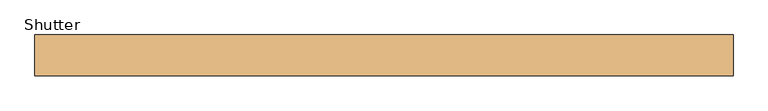
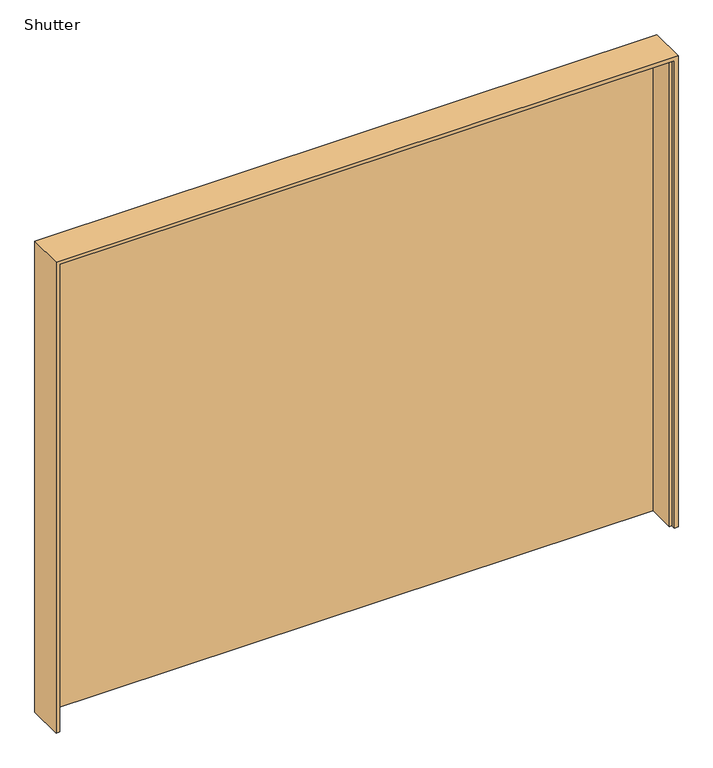
"""IFC4 building model written with IfcOpenShell, lengths in millimetres: door geometry, Shutter : H_DR_AMB_Roll up Door_Steel_W5000xH4000_Motorized."""

from ifc_helpers import new_model, si_unit, origin, origin_with_axes, place, context, project, spatial, polyline, outline, extrude, faceted_brep, source, transform, mapped, element, save


def shutter_f4e91935(model_context):
    return source(origin(), model_context, "Body", "SolidModel", [
        extrude(outline(polyline([(2470.0, 147.0), (2470.0, 112.0), (-2470.0, 112.0), (-2470.0, 147.0), (2470.0, 147.0)])), origin_with_axes(), (0.0, 0.0, 1.0), 3970.0),
        faceted_brep([(2470.0, 147.0, 0.0), (2500.0, 147.0, 0.0), (2500.0, -147.0, 0.0), (2470.0, -147.0, 0.0), (2470.0, -112.0, 0.0), (2450.0, -112.0, 0.0), (2450.0, 112.0, 0.0), (2470.0, 112.0, 0.0), (2470.0, 147.0, 3970.0), (-2470.0, 147.0, 3970.0), (-2470.0, 147.0, 0.0), (-2500.0, 147.0, 0.0), (-2500.0, 147.0, 4000.0), (2500.0, 147.0, 4000.0), (2500.0, -147.0, 4000.0), (-2500.0, -147.0, 4000.0), (-2500.0, -147.0, 0.0), (-2470.0, -147.0, 0.0), (-2470.0, -147.0, 3970.0), (2470.0, -147.0, 3970.0), (2470.0, -112.0, 3970.0), (-2470.0, -112.0, 3970.0), (-2470.0, -112.0, 0.0), (-2450.0, -112.0, 0.0), (-2450.0, -112.0, 3950.0), (2450.0, -112.0, 3950.0), (2450.0, 112.0, 3950.0), (-2450.0, 112.0, 3950.0), (-2450.0, 112.0, 0.0), (-2470.0, 112.0, 0.0), (-2470.0, 112.0, 3970.0), (2470.0, 112.0, 3970.0)], [[[0, 1, 2, 3, 4, 5, 6, 7]], [[1, 0, 8, 9, 10, 11, 12, 13]], [[2, 1, 13, 14]], [[3, 2, 14, 15, 16, 17, 18, 19]], [[4, 3, 19, 20]], [[5, 4, 20, 21, 22, 23, 24, 25]], [[6, 5, 25, 26]], [[7, 6, 26, 27, 28, 29, 30, 31]], [[0, 7, 31, 8]], [[9, 30, 29, 10]], [[10, 29, 28, 23, 22, 17, 16, 11]], [[15, 12, 11, 16]], [[21, 18, 17, 22]], [[27, 24, 23, 28]], [[8, 31, 30, 9]], [[14, 13, 12, 15]], [[20, 19, 18, 21]], [[26, 25, 24, 27]]]),
    ])


if __name__ == "__main__":
    model = new_model("IFC4")
    model_context = context("Model", 3, world=origin())
    ifc_project = project(units=[si_unit("LENGTHUNIT", "METRE", prefix="MILLI")], contexts=[model_context])
    site = spatial("IfcSite", under=ifc_project)
    building = spatial("IfcBuilding", under=site)
    placement = place(None, origin())
    shutter_shape = shutter_f4e91935(model_context)
    element("IfcDoor", 1, ObjectType="Shutter : H_DR_AMB_Roll up Door_Steel_W5000xH4000_Motorized", at=placement, inside=building, context=model_context, shape_type="MappedRepresentation", body=[
        mapped(shutter_shape, transform((0.0, 0.0, 0.0), x_axis=(1.0, 0.0, 0.0), y_axis=(0.0, 1.0, 0.0), z_axis=(0.0, 0.0, 1.0))),
    ])
    save(model, "model.ifc")

# Revit data of these elements
# Type "Shutter : H_DR_AMB_Roll up Door_Steel_W5000xH4000_Motorized"
#   Type Mark = "363"
#   Analytic Construction = "<None>"
#   프레임 투영 외부. = 25 mm
#   프레임 투영 내부. = 25 mm
#   프레임 폭 = 75 mm
#   Height = 4000 mm
#   Width = 5000 mm
#   Define Thermal Properties by = 1
#   문 패널 = none
#   문 프레임 = none
#   Function = (empty or 0)
#   Wall Closure = (empty or 0)
